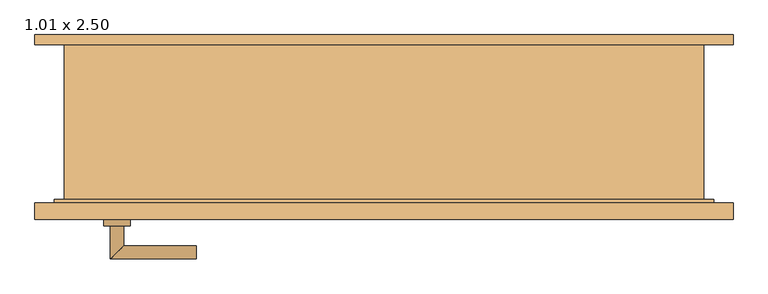
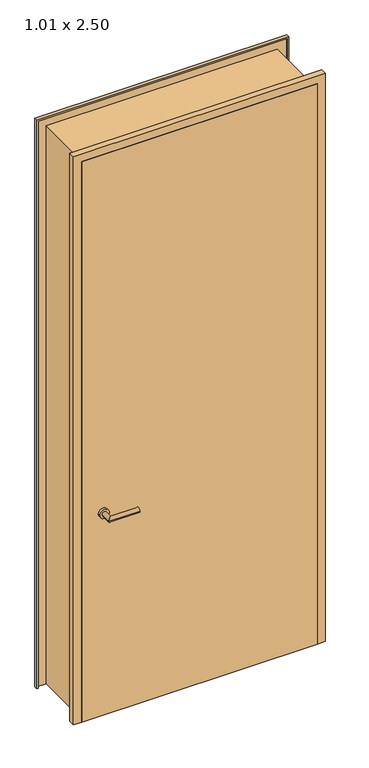
"""IFC4 building model written with IfcOpenShell, lengths in millimetres: door geometry, Drehflügel 1-flg - Stahlzarge : 1.01 x 2.50."""

from ifc_helpers import new_model, si_unit, point, frame, frame_2d, origin, place, context, project, spatial, polyline, circle_curve, ellipse_curve, trimmed, segment, composite_curve, outline, extrude, faceted_brep, source, transform, mapped, element, save
from ifc_brep_helpers import plane_surface, cylinder_surface, advanced_brep


def door_1_01_x_2_50_fbbdfe28(model_context):
    return source(origin(), model_context, "Body", "SolidModel", [
        advanced_brep(
        [(-415.0, -109.4346141, 1000.0), (-395.0, -109.4346141, 1000.0), (-395.0, -59.4346141, 1000.0), (-415.0, -39.4346141, 1000.0), (-285.0, -39.4346141, 1000.0), (-285.0, -59.4346141, 1000.0)],
        [
            (0, 1, circle_curve(frame((-405.0, -109.4346141, 1000.0), z_axis=(0.0, -1.0, 0.0), x_axis=(1.0, 0.0, 0.0)), 10.0)),
            (1, 0, circle_curve(frame((-405.0, -109.4346141, 1000.0), z_axis=(0.0, -1.0, 0.0), x_axis=(1.0, 0.0, 0.0)), 10.0)),
            (1, 2),
            (2, 3, ellipse_curve(frame((-405.0, -49.4346141, 1000.0), z_axis=(-0.7071067811865385, -0.7071067811865565, 0.0), x_axis=(0.7071067811865563, -0.7071067811865386, 0.0)), 14.1421356, 10.0)),
            (3, 0),
            (3, 2, ellipse_curve(frame((-405.0, -49.4346141, 1000.0), z_axis=(-0.7071067811865385, -0.7071067811865565, 0.0), x_axis=(0.7071067811865563, -0.7071067811865386, 0.0)), 14.1421356, 10.0)),
            (4, 5, circle_curve(frame((-285.0, -49.4346141, 1000.0), z_axis=(1.0, 0.0, 0.0), x_axis=(0.0, -1.0, 0.0)), 10.0)),
            (5, 4, circle_curve(frame((-285.0, -49.4346141, 1000.0), z_axis=(1.0, 0.0, 0.0), x_axis=(0.0, -1.0, 0.0)), 10.0)),
            (2, 5),
            (4, 3),
        ],
        [
            plane_surface(frame((-405.0, -109.4346141, -287.7526403), z_axis=(0.0, -1.0, 0.0), x_axis=(0.0, 0.0, 1.0))),
            cylinder_surface(frame((-405.0, -109.4346141, 1000.0), z_axis=(0.0, -1.0, 0.0), x_axis=(1.0, 0.0, 0.0)), 10.0),
            plane_surface(frame((-285.0, -49.4346141, -287.7526403), z_axis=(1.0, 0.0, 0.0), x_axis=(0.0, 0.0, 1.0))),
            cylinder_surface(frame((-405.0, -49.4346141, 1000.0), z_axis=(-1.0, 0.0, 0.0), x_axis=(0.0, -1.0, 0.0)), 10.0),
        ],
        [
            (0, [[1, 2]]),
            (1, [[3, 4, 5, -2]]),
            (1, [[-5, 6, -3, -1]]),
            (2, [[7, 8]]),
            (3, [[9, -7, 10, -4]]),
            (3, [[-10, -8, -9, -6]]),
        ],
    ),
        advanced_brep(
        [(-395.0, -169.4346141, 1000.0), (-415.0, -169.4346141, 1000.0), (-415.0, -219.4346141, 1000.0), (-395.0, -199.4346141, 1000.0), (-285.0, -199.4346141, 1000.0), (-285.0, -219.4346141, 1000.0)],
        [
            (0, 1, circle_curve(frame((-405.0, -169.4346141, 1000.0), z_axis=(0.0, 1.0, 0.0), x_axis=(-1.0, 0.0, 0.0)), 10.0)),
            (1, 0, circle_curve(frame((-405.0, -169.4346141, 1000.0), z_axis=(0.0, 1.0, 0.0), x_axis=(-1.0, 0.0, 0.0)), 10.0)),
            (1, 2),
            (2, 3, ellipse_curve(frame((-405.0, -209.4346141, 1000.0), z_axis=(-0.7071067811865475, 0.7071067811865475, 0.0), x_axis=(0.7071067811865474, 0.7071067811865476, 0.0)), 14.1421356, 10.0)),
            (3, 0),
            (3, 2, ellipse_curve(frame((-405.0, -209.4346141, 1000.0), z_axis=(-0.7071067811865475, 0.7071067811865475, 0.0), x_axis=(0.7071067811865474, 0.7071067811865476, 0.0)), 14.1421356, 10.0)),
            (4, 5, circle_curve(frame((-285.0, -209.4346141, 1000.0), z_axis=(1.0, 0.0, 0.0), x_axis=(0.0, -1.0, 0.0)), 10.0)),
            (5, 4, circle_curve(frame((-285.0, -209.4346141, 1000.0), z_axis=(1.0, 0.0, 0.0), x_axis=(0.0, -1.0, 0.0)), 10.0)),
            (2, 5),
            (4, 3),
        ],
        [
            plane_surface(frame((-405.0, -169.4346141, -287.7526403), z_axis=(0.0, 1.0, 0.0), x_axis=(0.0, 0.0, 1.0))),
            cylinder_surface(frame((-405.0, -169.4346141, 1000.0), z_axis=(0.0, 1.0, 0.0), x_axis=(-1.0, 0.0, 0.0)), 10.0),
            plane_surface(frame((-285.0, -209.4346141, -287.7526403), z_axis=(1.0, 0.0, 0.0), x_axis=(0.0, 0.0, 1.0))),
            cylinder_surface(frame((-405.0, -209.4346141, 1000.0), z_axis=(-1.0, 0.0, 0.0), x_axis=(0.0, -1.0, 0.0)), 10.0),
        ],
        [
            (0, [[1, 2]]),
            (1, [[3, 4, 5, -2]]),
            (1, [[-5, 6, -3, -1]]),
            (2, [[7, 8]]),
            (3, [[9, -7, 10, -4]]),
            (3, [[-10, -8, -9, -6]]),
        ],
    ),
        extrude(outline(composite_curve([segment(trimmed(circle_curve(frame_2d((1000.0, -405.0)), 20.0), [point((1000.0, -425.0))], [point((1000.0, -385.0))], False, "CARTESIAN"), True, "CONTINUOUS"), segment(trimmed(circle_curve(frame_2d((1000.0, -405.0)), 20.0), [point((1000.0, -385.0))], [point((1000.0, -425.0))], False, "CARTESIAN"), True, "CONTINUOUS")], self_intersect=False)), frame((0.0, -109.4346141, 0.0), z_axis=(0.0, 1.0, 0.0), x_axis=(0.0, 0.0, 1.0)), (0.0, 0.0, 1.0), 10.0),
        extrude(outline(composite_curve([segment(trimmed(circle_curve(frame_2d((1000.0, -405.0)), 20.0), [point((1000.0, -425.0))], [point((1000.0, -385.0))], False, "CARTESIAN"), True, "CONTINUOUS"), segment(trimmed(circle_curve(frame_2d((1000.0, -405.0)), 20.0), [point((1000.0, -385.0))], [point((1000.0, -425.0))], False, "CARTESIAN"), True, "CONTINUOUS")], self_intersect=False)), frame((0.0, -169.4346141, 0.0), z_axis=(0.0, 1.0, 0.0), x_axis=(0.0, 0.0, 1.0)), (0.0, 0.0, 1.0), 10.0),
        extrude(outline(polyline([(495.0, -134.4346141), (495.0, -159.4346141), (-495.0, -159.4346141), (-495.0, -134.4346141), (495.0, -134.4346141)])), frame((0.0, 0.0, 100.0), z_axis=(0.0, 0.0, 1.0), x_axis=(1.0, 0.0, 0.0)), (0.0, 0.0, 1.0), 2490.0),
        faceted_brep([(529.4603207, 120.5653859, 100.0), (529.4603207, 105.5653859, 100.0), (524.4603207, 105.5653859, 100.0), (524.4603207, 115.5653859, 100.0), (485.0, 115.5653859, 100.0), (485.0, -129.4346141, 100.0), (500.0, -129.4346141, 100.0), (500.0, -154.4346141, 100.0), (524.4603207, -154.4346141, 100.0), (524.4603207, -134.4346141, 100.0), (529.4603207, -134.4346141, 100.0), (529.4603207, -159.4346141, 100.0), (495.0, -159.4346141, 100.0), (495.0, -134.4346141, 100.0), (480.0, -134.4346141, 100.0), (480.0, 120.5653859, 100.0), (480.0, 120.5653859, 2575.0), (-480.0, 120.5653859, 2575.0), (-480.0, 120.5653859, 100.0), (-529.4603207, 120.5653859, 100.0), (-529.4603207, 120.5653859, 2624.4603207), (529.4603207, 120.5653859, 2624.4603207), (480.0, -134.4346141, 2575.0), (495.0, -134.4346141, 2590.0), (-495.0, -134.4346141, 2590.0), (-495.0, -134.4346141, 100.0), (-480.0, -134.4346141, 100.0), (-480.0, -134.4346141, 2575.0), (495.0, -159.4346141, 2590.0), (529.4603207, -159.4346141, 2624.4603207), (-529.4603207, -159.4346141, 2624.4603207), (-529.4603207, -159.4346141, 100.0), (-495.0, -159.4346141, 100.0), (-495.0, -159.4346141, 2590.0), (529.4603207, -134.4346141, 2624.4603207), (524.4603207, -134.4346141, 2619.4603207), (-524.4603207, -134.4346141, 2619.4603207), (-524.4603207, -134.4346141, 100.0), (-529.4603207, -134.4346141, 100.0), (-529.4603207, -134.4346141, 2624.4603207), (524.4603207, -154.4346141, 2619.4603207), (500.0, -154.4346141, 2595.0), (-500.0, -154.4346141, 2595.0), (-500.0, -154.4346141, 100.0), (-524.4603207, -154.4346141, 100.0), (-524.4603207, -154.4346141, 2619.4603207), (500.0, -129.4346141, 2595.0), (485.0, -129.4346141, 2580.0), (-485.0, -129.4346141, 2580.0), (-485.0, -129.4346141, 100.0), (-500.0, -129.4346141, 100.0), (-500.0, -129.4346141, 2595.0), (485.0, 115.5653859, 2580.0), (524.4603207, 115.5653859, 2619.4603207), (-524.4603207, 115.5653859, 2619.4603207), (-524.4603207, 115.5653859, 100.0), (-485.0, 115.5653859, 100.0), (-485.0, 115.5653859, 2580.0), (524.4603207, 105.5653859, 2619.4603207), (529.4603207, 105.5653859, 2624.4603207), (-529.4603207, 105.5653859, 2624.4603207), (-529.4603207, 105.5653859, 100.0), (-524.4603207, 105.5653859, 100.0), (-524.4603207, 105.5653859, 2619.4603207)], [[[0, 1, 2, 3, 4, 5, 6, 7, 8, 9, 10, 11, 12, 13, 14, 15]], [[15, 16, 17, 18, 19, 20, 21, 0]], [[14, 22, 16, 15]], [[13, 23, 24, 25, 26, 27, 22, 14]], [[12, 28, 23, 13]], [[11, 29, 30, 31, 32, 33, 28, 12]], [[10, 34, 29, 11]], [[9, 35, 36, 37, 38, 39, 34, 10]], [[8, 40, 35, 9]], [[7, 41, 42, 43, 44, 45, 40, 8]], [[6, 46, 41, 7]], [[5, 47, 48, 49, 50, 51, 46, 6]], [[4, 52, 47, 5]], [[3, 53, 54, 55, 56, 57, 52, 4]], [[2, 58, 53, 3]], [[1, 59, 60, 61, 62, 63, 58, 2]], [[0, 21, 59, 1]], [[20, 19, 61, 60]], [[19, 18, 26, 25, 32, 31, 38, 37, 44, 43, 50, 49, 56, 55, 62, 61]], [[27, 26, 18, 17]], [[33, 32, 25, 24]], [[39, 38, 31, 30]], [[45, 44, 37, 36]], [[51, 50, 43, 42]], [[57, 56, 49, 48]], [[63, 62, 55, 54]], [[22, 27, 17, 16]], [[28, 33, 24, 23]], [[34, 39, 30, 29]], [[40, 45, 36, 35]], [[46, 51, 42, 41]], [[52, 57, 48, 47]], [[58, 63, 54, 53]], [[21, 20, 60, 59]]]),
    ])


if __name__ == "__main__":
    model = new_model("IFC4")
    model_context = context("Model", 3, world=origin())
    ifc_project = project(units=[si_unit("LENGTHUNIT", "METRE", prefix="MILLI")], contexts=[model_context])
    site = spatial("IfcSite", under=ifc_project)
    building = spatial("IfcBuilding", under=site)
    placement = place(None, origin())
    door_1_01_x_2_50_shape = door_1_01_x_2_50_fbbdfe28(model_context)
    element("IfcDoor", 1, ObjectType="Drehflügel 1-flg - Stahlzarge : 1.01 x 2.50", at=placement, inside=building, context=model_context, shape_type="MappedRepresentation", body=[
        mapped(door_1_01_x_2_50_shape, transform((0.0, 0.0, 0.0), x_axis=(1.0, 0.0, 0.0), y_axis=(0.0, 1.0, 0.0), z_axis=(0.0, 0.0, 1.0))),
    ])
    save(model, "model.ifc")

# Revit data of these elements
# Type "Drehflügel 1-flg - Stahlzarge : 1.01 x 2.50"
#   Type Mark = "29"
#   Operation = "SingleSwingRight"
#   Keynote = "16.03"
#   Analytic Construction = "Metall"
#   Thermal Resistance (R) = 0.270117 (m²·K)/W
#   Heat Transfer Coefficient (U) = 3.7021 W/(m²·K)
#   Rough Width = 1.010 m
#   Rough Height [instance default] = 2.600 m
#   Höhe Türgriff [instance default] = 0.900 m
#   Height = 2.500 m
#   Fußbodenaufbau [instance default] = 0.100 m
#   Width = 1.010 m
#   Sichtbarkeit Sturzlinien [instance default] = yes
#   Türgriff auswählen [instance default] = element 221079
#   Türgriff [instance default] = none
#   Türflügel [instance default] = none
#   Rahmen/Pfosten [instance default] = Metall - Lackiert - Grau
#   Visual Light Transmittance = 0
#   Solar Heat Gain Coefficient = 0
#   Function = (empty or 0)
#   Wall Closure = (empty or 0)
# Element 1 (IfcDoor, "Drehflügel 1-flg - Stahlzarge : 1.01 x 2.50")
#   Materials on its faces: "Metall - Lackiert - Grau", "Metall - Chrom", "Holz - Birke"
# Materials
#   "Metall - Lackiert - Grau": class "Farbe 1", colour RGB 98 98 98, transparency 0, Cost = 0
#   "Metall - Chrom": class "Metall", colour RGB 247 247 247, transparency 0, Cost = 0
#   "Holz - Birke": class "Holz", colour RGB 213 164 103, transparency 0, Cost = 0
